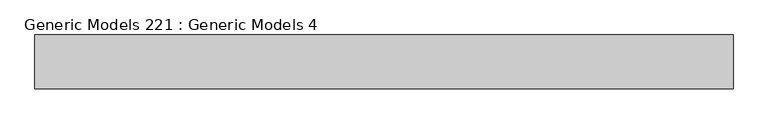
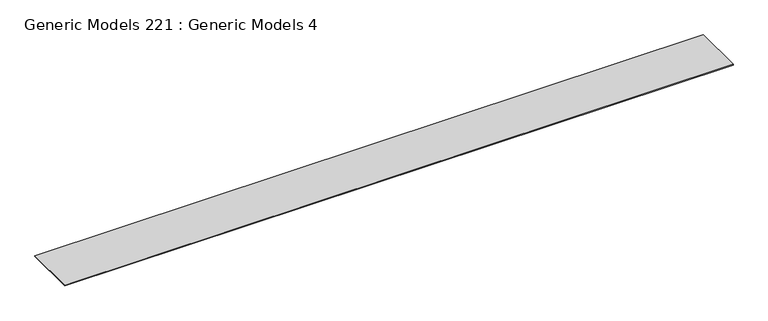
"""IFC4 building model written with IfcOpenShell, lengths in millimetres: proxy geometry, Generic Models 221 : Generic Models 4."""

from ifc_helpers import new_model, si_unit, frame, origin, place, context, project, spatial, polyline, outline, extrude, source, transform, mapped, element, save


def generic_models_221_generic_models_4_8be4d322(model_context):
    return source(origin(), model_context, "Body", "SweptSolid", [
        extrude(outline(polyline([(-2152.1733045, -29182.8735041), (-2152.1733045, -30617.9735041), (-20795.7733045, -30617.9735041), (-20795.7733045, -29182.8735041), (-2152.1733045, -29182.8735041)])), frame((0.0, 0.0, 126809.246), z_axis=(0.0, 0.0, 1.0), x_axis=(1.0, 0.0, 0.0)), (0.0, 0.0, 1.0), 19.05),
    ])


if __name__ == "__main__":
    model = new_model("IFC4")
    model_context = context("Model", 3, world=origin())
    ifc_project = project(units=[si_unit("LENGTHUNIT", "METRE", prefix="MILLI")], contexts=[model_context])
    site = spatial("IfcSite", under=ifc_project)
    building = spatial("IfcBuilding", under=site)
    placement = place(None, origin())
    generic_models_221_generic_models_4_shape = generic_models_221_generic_models_4_8be4d322(model_context)
    element("IfcBuildingElementProxy", 1, Name="Generic Models 221 : Generic Models 4", ObjectType="Generic Models 221 : Generic Models 4", at=placement, inside=building, context=model_context, shape_type="MappedRepresentation", body=[
        mapped(generic_models_221_generic_models_4_shape, transform((0.0, 0.0, 0.0), x_axis=(1.0, 0.0, 0.0), y_axis=(0.0, 1.0, 0.0), z_axis=(0.0, 0.0, 1.0))),
    ])
    save(model, "model.ifc")

# Revit data of these elements
# Element 1 (IfcBuildingElementProxy, "Generic Models 221 : Generic Models 4")
#   Materials on its faces: "_CDX PLYWOOD - SEE STRUCT DWGs"
# Materials
#   "_CDX PLYWOOD - SEE STRUCT DWGs": class "Generic", colour RGB 98 75 74, transparency 0, Cost = 0
